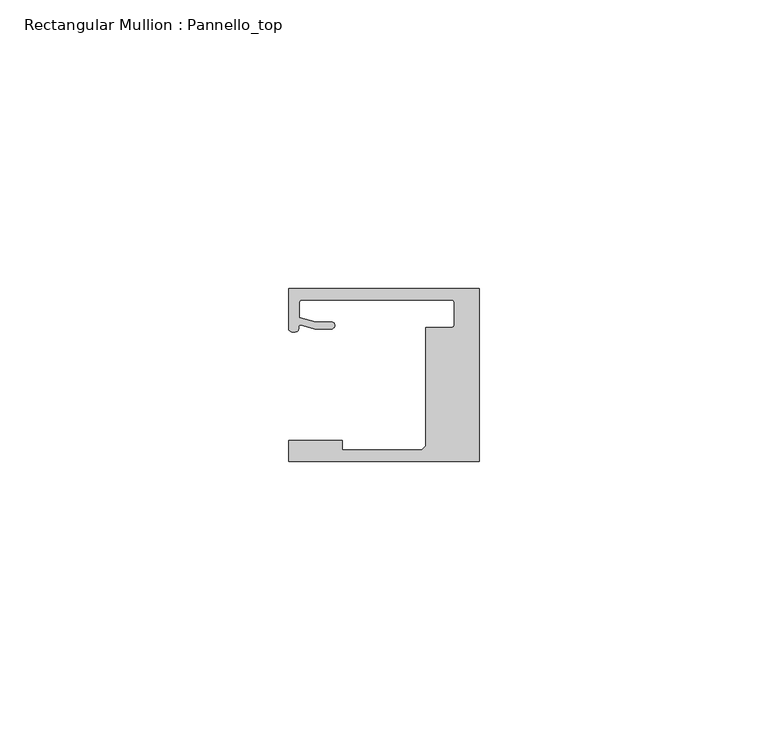
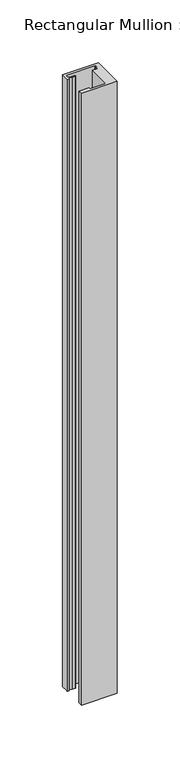
"""IFC4 building model written with IfcOpenShell, lengths in millimetres: member geometry, Rectangular Mullion : Pannello_top."""

import ifcopenshell
import ifcopenshell.guid

model = None  # the IFC model being written
_history = None  # IfcOwnerHistory: only IFC2X3 demands one
_inside = {}  # id of a spatial element -> (the spatial element, [elements in it])
_under = {}  # id of a project, library or spatial element -> (it, [spatial elements below it])
_declared = {}  # id of a project -> (the project, [libraries it declares])
_typed = {}  # id of a type object -> (the type object, [elements of that type])
_made_of = {}  # id of a material, layer set ... -> (it, [elements and type objects made of it])


def new_model(schema):
    """Start an empty IFC model of exactly this schema.

    Asked for "IFC4X3", IfcOpenShell would pick the latest addendum, in which some entities
    have other attributes; the version numbers below select the first issue.
    IFC2X3 requires an IfcOwnerHistory on every rooted entity: one is made here for all.
    """
    global model, _history
    if schema == "IFC4X3":
        model = ifcopenshell.file(schema_version=(4, 3, 0, 0))
    else:
        model = ifcopenshell.file(schema=schema)
    _inside.clear()
    _under.clear()
    _declared.clear()
    _typed.clear()
    _made_of.clear()
    _history = None
    if model.schema == "IFC2X3":
        org = make("IfcOrganization", Name="unknown")
        user = make(
            "IfcPersonAndOrganization",
            ThePerson=make("IfcPerson", FamilyName="unknown"),
            TheOrganization=org,
        )
        app = make(
            "IfcApplication",
            ApplicationDeveloper=org,
            Version="unknown",
            ApplicationFullName="unknown",
            ApplicationIdentifier="unknown",
        )
        _history = make(
            "IfcOwnerHistory",
            OwningUser=user,
            OwningApplication=app,
            ChangeAction="ADDED",
            CreationDate=0,
        )
    return model


def make(cls, **values):
    """One entity of the class cls with the attributes given. An attribute that is None is left unset."""
    return model.create_entity(
        cls, **{name: value for name, value in values.items() if value is not None}
    )


def rooted(cls, **values):
    """An entity with a GlobalId (a new one), such as an element, a storey or a relation."""
    return make(cls, GlobalId=ifcopenshell.guid.new(), OwnerHistory=_history, **values)


def si_unit(unit_type, name, prefix=None):
    """IfcSIUnit, for example si_unit("LENGTHUNIT", "METRE", prefix="MILLI")."""
    return make("IfcSIUnit", UnitType=unit_type, Prefix=prefix, Name=name)


def assignment(units):
    """IfcUnitAssignment: the units of a project."""
    return None if units is None else make("IfcUnitAssignment", Units=units)


def point(xyz):
    """IfcCartesianPoint."""
    return None if xyz is None else make("IfcCartesianPoint", Coordinates=xyz)


def direction(xyz):
    """IfcDirection."""
    return None if xyz is None else make("IfcDirection", DirectionRatios=xyz)


def frame(location, z_axis=None, x_axis=None):
    """IfcAxis2Placement3D, a coordinate frame: its origin and axes. An axis left out is left unset."""
    return make(
        "IfcAxis2Placement3D",
        Location=point(location),
        Axis=direction(z_axis),
        RefDirection=direction(x_axis),
    )


def origin():
    """The frame at (0, 0, 0) with its axes left unset."""
    return frame((0.0, 0.0, 0.0))


def place(relative_to, where):
    """IfcLocalPlacement: puts the frame where relative to a parent placement (None: the world)."""
    return make(
        "IfcLocalPlacement", PlacementRelTo=relative_to, RelativePlacement=where
    )


def context(
    kind, dimensions, precision=None, world=None, true_north=None, identifier=None
):
    """IfcGeometricRepresentationContext, for example the 3D "Model" context."""
    return make(
        "IfcGeometricRepresentationContext",
        ContextIdentifier=identifier,
        ContextType=kind,
        CoordinateSpaceDimension=dimensions,
        Precision=precision,
        WorldCoordinateSystem=world,
        TrueNorth=true_north,
    )


def project(units=None, contexts=None):
    """IfcProject with its units and contexts."""
    return rooted(
        "IfcProject",
        Name="project",
        RepresentationContexts=contexts,
        UnitsInContext=assignment(units),
    )


def spatial(cls, under=None, at=None, **own):
    """A site, building, storey or space (cls), placed at a placement, below another one or the project."""
    s = rooted(cls, ObjectPlacement=at, **own)
    if under is not None:
        _under.setdefault(under.id(), (under, []))[1].append(s)
    return s


def polyline(points):
    """IfcPolyline through the points."""
    return make("IfcPolyline", Points=[point(p) for p in points])


def circle_curve(where, radius):
    """IfcCircle in the frame where."""
    return make("IfcCircle", Position=where, Radius=radius)


def shape(context_of_items, identifier, shape_type, items):
    """IfcShapeRepresentation: the items that make up one representation, for example the "Body"."""
    return make(
        "IfcShapeRepresentation",
        ContextOfItems=context_of_items,
        RepresentationIdentifier=identifier,
        RepresentationType=shape_type,
        Items=items,
    )


def source(mapping_origin, context_of_items, identifier, shape_type, items):
    """IfcRepresentationMap: a shape defined once, which mapped items show again and again."""
    return make(
        "IfcRepresentationMap",
        MappingOrigin=mapping_origin,
        MappedRepresentation=shape(context_of_items, identifier, shape_type, items),
    )


def transform(
    local_origin,
    x_axis=None,
    y_axis=None,
    z_axis=None,
    scale=None,
    scale2=None,
    scale3=None,
    uniform=True,
):
    """IfcCartesianTransformationOperator3D, or its non-uniform kind. x_axis, y_axis, z_axis: its Axis1, 2, 3."""
    if uniform:
        return make(
            "IfcCartesianTransformationOperator3D",
            Axis1=direction(x_axis),
            Axis2=direction(y_axis),
            LocalOrigin=point(local_origin),
            Scale=scale,
            Axis3=direction(z_axis),
        )
    return make(
        "IfcCartesianTransformationOperator3DnonUniform",
        Axis1=direction(x_axis),
        Axis2=direction(y_axis),
        LocalOrigin=point(local_origin),
        Scale=scale,
        Axis3=direction(z_axis),
        Scale2=scale2,
        Scale3=scale3,
    )


def mapped(mapping_source, mapping_target):
    """IfcMappedItem: shows the shape of a source again, moved by a transform."""
    return make(
        "IfcMappedItem", MappingSource=mapping_source, MappingTarget=mapping_target
    )


def made_of(thing, what):
    """Note that an element or type object is made of a material, layer set ...; save() writes the relation."""
    if what is not None:
        _made_of.setdefault(what.id(), (what, []))[1].append(thing)
    return thing


def element(
    cls,
    number,
    at=None,
    inside=None,
    cuts=None,
    type_object=None,
    material=None,
    context=None,
    identifier="Body",
    shape_type=None,
    held_by="IfcProductDefinitionShape",
    body=None,
    shapes=None,
    **own,
):
    """One element of the class cls, such as IfcWall. Its Tag is "e" and its number.

    at: its placement. inside: the storey or other place that contains it. cuts: it is an
    opening in that element (IfcRelVoidsElement). A single representation is given by context,
    identifier, shape_type and body (its items); several are given by shapes. held_by: the class
    of the entity that holds the representations. save() writes the other relations.
    """
    e = rooted(cls, Tag="e%d" % number, ObjectPlacement=at, **own)
    if body is not None:
        shapes = [shape(context, identifier, shape_type, body)]
    if shapes is not None:
        e.Representation = make(held_by, Representations=shapes)
    if inside is not None:
        _inside.setdefault(inside.id(), (inside, []))[1].append(e)
    if cuts is not None:
        rooted(
            "IfcRelVoidsElement", RelatingBuildingElement=cuts, RelatedOpeningElement=e
        )
    if type_object is not None:
        _typed.setdefault(type_object.id(), (type_object, []))[1].append(e)
    return made_of(e, material)


def aggregate(whole, parts):
    """IfcRelAggregates: a whole, such as a stair, and the parts it consists of."""
    return rooted("IfcRelAggregates", RelatingObject=whole, RelatedObjects=parts)


def save(model, path):
    """Write the relations noted so far, then the file.

    IfcRelAggregates (storeys below a building ...), IfcRelContainedInSpatialStructure (elements
    in a storey), IfcRelDefinesByType, IfcRelAssociatesMaterial and IfcRelDeclares: one each for
    every whole, place, type object, material and project.
    """
    for whole, parts in _under.values():
        aggregate(whole, parts)
    for where, things in _inside.values():
        rooted(
            "IfcRelContainedInSpatialStructure",
            RelatedElements=things,
            RelatingStructure=where,
        )
    for kind, things in _typed.values():
        rooted("IfcRelDefinesByType", RelatedObjects=things, RelatingType=kind)
    for what, things in _made_of.values():
        rooted("IfcRelAssociatesMaterial", RelatedObjects=things, RelatingMaterial=what)
    for by, libraries in _declared.values():
        rooted("IfcRelDeclares", RelatingContext=by, RelatedDefinitions=libraries)
    model.write(path)


def plane_surface(at):
    """IfcPlane: the flat surface through the origin of the frame at, square to its z axis."""
    return make("IfcPlane", Position=at)


def cylinder_surface(at, radius):
    """IfcCylindricalSurface: all points at the distance radius from the z axis of the frame at."""
    return make("IfcCylindricalSurface", Position=at, Radius=radius)


def revolved_surface(curve, axis_point, axis_direction):
    """IfcSurfaceOfRevolution: the curve turned about the line through axis_point along axis_direction."""
    return make(
        "IfcSurfaceOfRevolution",
        SweptCurve=make("IfcArbitraryOpenProfileDef", ProfileType="CURVE", Curve=curve),
        AxisPosition=make("IfcAxis1Placement", Location=point(axis_point), Axis=direction(axis_direction)),
    )


def extruded_surface(curve, direction_of_extrusion, depth):
    """IfcSurfaceOfLinearExtrusion: the curve pushed along a direction by depth."""
    return make(
        "IfcSurfaceOfLinearExtrusion",
        SweptCurve=make("IfcArbitraryOpenProfileDef", ProfileType="CURVE", Curve=curve),
        ExtrudedDirection=direction(direction_of_extrusion),
        Depth=depth,
    )


def spline_curve(degree, points, multiplicities, knots, weights=None):
    """IfcBSplineCurveWithKnots; with weights, IfcRationalBSplineCurveWithKnots."""
    own = dict(
        Degree=degree,
        ControlPointsList=[point(p) for p in points],
        CurveForm="UNSPECIFIED",
        ClosedCurve=False,
        SelfIntersect=False,
        KnotMultiplicities=multiplicities,
        Knots=knots,
        KnotSpec="UNSPECIFIED",
    )
    if weights is None:
        return make("IfcBSplineCurveWithKnots", **own)
    return make("IfcRationalBSplineCurveWithKnots", WeightsData=weights, **own)


def advanced_brep(points, edges, surfaces, faces):
    """IfcAdvancedBrep: a solid bounded by faces that lie on surfaces and meet in shared edges.

    An edge is (start, end): straight between two places in points (the first is 0);
    or (start, end, curve); or (start, end, curve, False) where it runs against its curve.
    A face is (place in surfaces, loops), or (place, loops, False) where it looks against
    its surface's normal. A loop lists edges by number (the first is 1), with a minus sign
    where the edge is run from its end to its start. The first loop is the outer one.
    """
    corners = [point(p) for p in points]
    vertices = [make("IfcVertexPoint", VertexGeometry=c) for c in corners]
    made = []
    for start, end, *more in edges:
        made.append(
            make(
                "IfcEdgeCurve",
                EdgeStart=vertices[start],
                EdgeEnd=vertices[end],
                EdgeGeometry=more[0] if more else make("IfcPolyline", Points=[corners[start], corners[end]]),
                SameSense=more[1] if len(more) > 1 else True,
            )
        )
    hull = []
    for where, loops, *sense in faces:
        bounds = []
        for j, loop in enumerate(loops):
            ring = [make("IfcOrientedEdge", EdgeElement=made[abs(k) - 1], Orientation=k > 0) for k in loop]
            bounds.append(
                make(
                    "IfcFaceOuterBound" if j == 0 else "IfcFaceBound",
                    Bound=make("IfcEdgeLoop", EdgeList=ring),
                    Orientation=True,
                )
            )
        hull.append(make("IfcAdvancedFace", Bounds=bounds, FaceSurface=surfaces[where], SameSense=sense[0] if sense else True))
    return make("IfcAdvancedBrep", Outer=make("IfcClosedShell", CfsFaces=hull))


def rectangular_mullion_pannello_top_2eeb697f(model_context):
    return source(origin(), model_context, "Body", "AdvancedBrep", [
        advanced_brep(
        [(-33.0, -15.0, 0.0), (0.0, -15.0, 0.0), (0.0, 15.0, 0.0), (-33.0000135, 15.0, 0.0), (-33.0000135, 8.0000472, 0.0), (-30.9223017, 8.6490241, 0.0), (-28.4999305, 7.9999523, 0.0), (-25.59998, 7.9999523, 0.0), (-25.59998, 9.1999523, 0.0), (-28.3419477, 9.1999523, 0.0), (-31.19998, 9.9657591, 0.0), (-31.19998, 12.50001, 0.0), (-30.69998, 13.00001, 0.0), (-4.7999726, 13.00001, 0.0), (-4.2999726, 12.50001, 0.0), (-4.2999726, 8.7500595, 0.0), (-4.7999726, 8.2500595, 0.0), (-9.2999726, 8.2500595, 0.0), (-9.2999726, -12.2999849, 0.0), (-10.0000103, -13.0000004, 0.0), (-23.700041, -13.0000004, 0.0), (-23.700041, -11.3000004, 0.0), (-33.0, -11.3000004, 0.0), (-33.0, -15.0, -595.0), (-33.0, -11.3000004, -595.0), (-23.700041, -11.3000004, -595.0), (-23.700041, -13.0000004, -595.0), (-10.0000103, -13.0000004, -595.0), (-9.2999726, -12.2999849, -595.0), (-9.2999726, 8.2500595, -595.0), (-4.7999726, 8.2500595, -595.0), (-4.2999726, 8.7500595, -595.0), (-4.2999726, 12.50001, -595.0), (-4.7999726, 13.00001, -595.0), (-30.69998, 13.00001, -595.0), (-31.19998, 12.50001, -595.0), (-31.19998, 9.9657591, -595.0), (-28.3419477, 9.1999523, -595.0), (-25.59998, 9.1999523, -595.0), (-25.59998, 7.9999523, -595.0), (-28.4999305, 7.9999523, -595.0), (-30.9223017, 8.6490241, -595.0), (-33.0000135, 8.0000472, -595.0), (-33.0000135, 15.0, -595.0), (0.0, 15.0, -595.0), (0.0, -15.0, -595.0)],
        [
            (0, 1),
            (1, 2),
            (2, 3),
            (3, 4),
            (4, 5, spline_curve(3, [(-33.0000135, 8.0000472, 0.0), (-33.0000135, 7.457047519, 0.0), (-32.262327879, 7.456527435, 0.0), (-31.357433266, 7.563996614, 0.0), (-31.305645054, 7.690065204, 0.0), (-31.298563602, 8.366228555, 0.0), (-31.312054066, 8.717747958, 0.0), (-30.9223017, 8.6490241, 0.0)], [4, 2, 2, 4], [0.0, 0.0027053965905959043, 0.0058611956533709, 0.007702013405570312])),
            (5, 6),
            (6, 7),
            (7, 8, circle_curve(frame((-25.59998, 8.5999523, 0.0), z_axis=(0.0, 0.0, 1.0), x_axis=(0.0, 1.0, 0.0)), 0.6)),
            (8, 9),
            (9, 10),
            (10, 11),
            (11, 12, circle_curve(frame((-30.69998, 12.50001, 0.0), z_axis=(0.0, 0.0, -1.0), x_axis=(0.0, 1.0, 0.0)), 0.5)),
            (12, 13),
            (13, 14, circle_curve(frame((-4.7999726, 12.50001, 0.0), z_axis=(0.0, 0.0, -1.0), x_axis=(1.0, 0.0, 0.0)), 0.5)),
            (14, 15),
            (15, 16, circle_curve(frame((-4.7999726, 8.7500595, 0.0), z_axis=(0.0, 0.0, -1.0), x_axis=(0.0, -1.0, 0.0)), 0.5)),
            (16, 17),
            (17, 18),
            (18, 19),
            (19, 20),
            (20, 21),
            (21, 22),
            (22, 0),
            (23, 24),
            (24, 25),
            (25, 26),
            (26, 27),
            (27, 28),
            (28, 29),
            (29, 30),
            (30, 31, circle_curve(frame((-4.7999726, 8.7500595, -595.0), z_axis=(0.0, 0.0, 1.0), x_axis=(0.0, -1.0, 0.0)), 0.5)),
            (31, 32),
            (32, 33, circle_curve(frame((-4.7999726, 12.50001, -595.0), z_axis=(0.0, 0.0, 1.0), x_axis=(1.0, 0.0, 0.0)), 0.5)),
            (33, 34),
            (34, 35, circle_curve(frame((-30.69998, 12.50001, -595.0), z_axis=(0.0, 0.0, 1.0), x_axis=(0.0, 1.0, 0.0)), 0.5)),
            (35, 36),
            (36, 37),
            (37, 38),
            (38, 39, circle_curve(frame((-25.59998, 8.5999523, -595.0), z_axis=(0.0, 0.0, -1.0), x_axis=(0.0, 1.0, 0.0)), 0.6)),
            (39, 40),
            (40, 41),
            (41, 42, spline_curve(3, [(-30.9223017, 8.6490241, -595.0), (-31.312054066, 8.717747958, -595.0), (-31.298563602, 8.366228555, -595.0), (-31.305645054, 7.690065204, -595.0), (-31.357433266, 7.563996614, -595.0), (-32.262327879, 7.456527435, -595.0), (-33.0000135, 7.457047519, -595.0), (-33.0000135, 8.0000472, -595.0)], [4, 2, 2, 4], [0.0, 0.001840817752199412, 0.004996616814974408, 0.007702013405570312])),
            (42, 43),
            (43, 44),
            (44, 45),
            (45, 23),
            (0, 23),
            (45, 1),
            (44, 2),
            (43, 3),
            (42, 4),
            (41, 5),
            (40, 6),
            (39, 7),
            (38, 8),
            (37, 9),
            (36, 10),
            (35, 11),
            (34, 12),
            (33, 13),
            (32, 14),
            (31, 15),
            (30, 16),
            (29, 17),
            (28, 18),
            (27, 19),
            (26, 20),
            (25, 21),
            (24, 22),
        ],
        [
            plane_surface(frame((0.0, -36.2491502, 0.0), z_axis=(0.0, 0.0, 1.0), x_axis=(-1.0, 0.0, 0.0))),
            plane_surface(frame((0.0, -36.2491502, -595.0), z_axis=(0.0, 0.0, -1.0), x_axis=(-1.0, 0.0, 0.0))),
            plane_surface(frame((-33.0, -15.0, 0.0), z_axis=(0.0, -1.0, 0.0), x_axis=(0.0, 0.0, -1.0))),
            plane_surface(frame((0.0, -15.0, 0.0), z_axis=(1.0, 0.0, 0.0), x_axis=(0.0, 0.0, -1.0))),
            plane_surface(frame((0.0, 15.0, 0.0), z_axis=(0.0, 1.0, 0.0), x_axis=(0.0, 0.0, -1.0))),
            plane_surface(frame((-33.0000135, 15.0, 0.0), z_axis=(-1.0, 0.0, 0.0), x_axis=(0.0, 0.0, -1.0))),
            extruded_surface(spline_curve(3, [(-33.0000135, 8.0000472, -595.0), (-33.0000135, 7.457047519, -595.0), (-32.262327879, 7.456527435, -595.0), (-31.357433266, 7.563996614, -595.0), (-31.305645054, 7.690065204, -595.0), (-31.298563602, 8.366228555, -595.0), (-31.312054066, 8.717747958, -595.0), (-30.9223017, 8.6490241, -595.0)], [4, 2, 2, 4], [0.0, 0.0027053965905959043, 0.0058611956533709, 0.007702013405570312]), (0.0, 0.0, 595.0), 595.0),
            plane_surface(frame((-30.9223017, 8.6490241, 0.0), z_axis=(-0.25881883200192934, -0.9659258833891746, 0.0), x_axis=(0.0, 0.0, -1.0))),
            plane_surface(frame((-28.4999305, 7.9999523, 0.0), z_axis=(0.0, -1.0, 0.0), x_axis=(0.0, 0.0, -1.0))),
            cylinder_surface(frame((-25.59998, 8.5999523, 0.0), z_axis=(0.0, 0.0, 1.0), x_axis=(0.0, 1.0, 0.0)), 0.6),
            plane_surface(frame((-25.59998, 9.1999523, 0.0), z_axis=(0.0, 1.0, 0.0), x_axis=(0.0, 0.0, -1.0))),
            plane_surface(frame((-28.3419477, 9.1999523, 0.0), z_axis=(0.25881883204288636, 0.9659258833782002, 0.0), x_axis=(0.0, 0.0, -1.0))),
            plane_surface(frame((-31.19998, 9.9657591, 0.0), z_axis=(1.0, 0.0, 0.0), x_axis=(0.0, 0.0, -1.0))),
            revolved_surface(polyline([(-30.69998, 13.00001, -595.0), (-30.69998, 13.00001, 0.0)]), (-30.69998, 12.50001, 0.0), (0.0, 0.0, -1.0)),
            plane_surface(frame((-30.69998, 13.00001, 0.0), z_axis=(0.0, -1.0, 0.0), x_axis=(0.0, 0.0, -1.0))),
            revolved_surface(polyline([(-4.2999726, 12.50001, -595.0), (-4.2999726, 12.50001, 0.0)]), (-4.7999726, 12.50001, 0.0), (0.0, 0.0, -1.0)),
            plane_surface(frame((-4.2999726, 12.50001, 0.0), z_axis=(-1.0, 0.0, 0.0), x_axis=(0.0, 0.0, -1.0))),
            revolved_surface(polyline([(-4.7999726, 8.2500595, -595.0), (-4.7999726, 8.2500595, 0.0)]), (-4.7999726, 8.7500595, 0.0), (0.0, 0.0, -1.0)),
            plane_surface(frame((-4.7999726, 8.2500595, 0.0), z_axis=(0.0, 1.0, 0.0), x_axis=(0.0, 0.0, -1.0))),
            plane_surface(frame((-9.2999726, 8.2500595, 0.0), z_axis=(-1.0, 0.0, 0.0), x_axis=(0.0, 0.0, -1.0))),
            plane_surface(frame((-9.2999726, -12.2999849, 0.0), z_axis=(-0.7070955486277984, 0.7071180135668678, 0.0), x_axis=(0.0, 0.0, -1.0))),
            plane_surface(frame((-10.0000103, -13.0000004, 0.0), z_axis=(0.0, 1.0, 0.0), x_axis=(0.0, 0.0, -1.0))),
            plane_surface(frame((-23.700041, -13.0000004, 0.0), z_axis=(1.0, 0.0, 0.0), x_axis=(0.0, 0.0, -1.0))),
            plane_surface(frame((-23.700041, -11.3000004, 0.0), z_axis=(0.0, 1.0, 0.0), x_axis=(0.0, 0.0, -1.0))),
            plane_surface(frame((-33.0, -11.3000004, 0.0), z_axis=(-1.0, 0.0, 0.0), x_axis=(0.0, 0.0, -1.0))),
        ],
        [
            (0, [[1, 2, 3, 4, 5, 6, 7, 8, 9, 10, 11, 12, 13, 14, 15, 16, 17, 18, 19, 20, 21, 22, 23]]),
            (1, [[24, 25, 26, 27, 28, 29, 30, 31, 32, 33, 34, 35, 36, 37, 38, 39, 40, 41, 42, 43, 44, 45, 46]]),
            (2, [[-1, 47, -46, 48]]),
            (3, [[-2, -48, -45, 49]]),
            (4, [[-3, -49, -44, 50]]),
            (5, [[-4, -50, -43, 51]]),
            (6, [[-5, -51, -42, 52]]),
            (7, [[-6, -52, -41, 53]]),
            (8, [[-7, -53, -40, 54]]),
            (9, [[-8, -54, -39, 55]]),
            (10, [[-9, -55, -38, 56]]),
            (11, [[-10, -56, -37, 57]]),
            (12, [[-11, -57, -36, 58]]),
            (13, [[-12, -58, -35, 59]]),
            (14, [[-13, -59, -34, 60]]),
            (15, [[-14, -60, -33, 61]]),
            (16, [[-15, -61, -32, 62]]),
            (17, [[-16, -62, -31, 63]]),
            (18, [[-17, -63, -30, 64]]),
            (19, [[-18, -64, -29, 65]]),
            (20, [[-19, -65, -28, 66]]),
            (21, [[-20, -66, -27, 67]]),
            (22, [[-21, -67, -26, 68]]),
            (23, [[-22, -68, -25, 69]]),
            (24, [[-23, -69, -24, -47]]),
        ],
    ),
    ])


if __name__ == "__main__":
    model = new_model("IFC4")
    model_context = context("Model", 3, world=origin())
    ifc_project = project(units=[si_unit("LENGTHUNIT", "METRE", prefix="MILLI")], contexts=[model_context])
    site = spatial("IfcSite", under=ifc_project)
    building = spatial("IfcBuilding", under=site)
    placement = place(None, origin())
    rectangular_mullion_pannello_top_shape = rectangular_mullion_pannello_top_2eeb697f(model_context)
    element("IfcMember", 1, ObjectType="Rectangular Mullion : Pannello_top", at=placement, inside=building, context=model_context, shape_type="MappedRepresentation", body=[
        mapped(rectangular_mullion_pannello_top_shape, transform((0.0, 0.0, 0.0), x_axis=(1.0, 0.0, 0.0), y_axis=(0.0, 1.0, 0.0), z_axis=(0.0, 0.0, 1.0))),
    ])
    save(model, "model.ifc")

# Revit data of these elements
# Type "Rectangular Mullion : Pannello_top"
#   built-in parameter 1007322 = 0.0984252 (stored number, unit not read)
#   built-in parameter 1007321 = 0 (stored number, unit not read)
#   built-in parameter 1007320 = 0.0305117 (stored number, unit not read)
